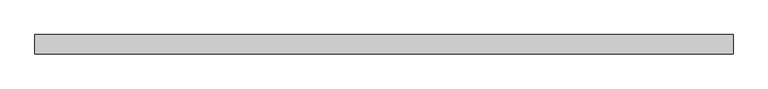
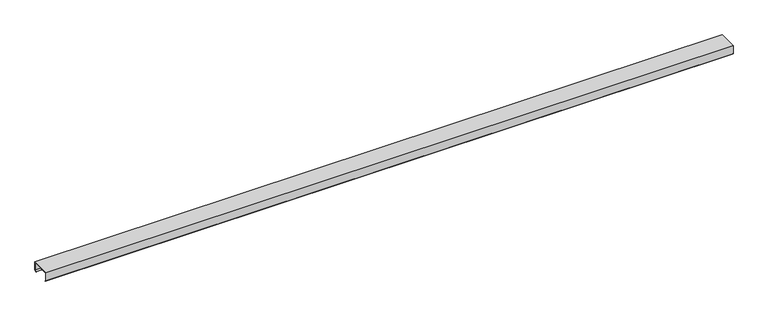
"""IFC4 building model written with IfcOpenShell, lengths in millimetres: proxy geometry, Generic Models 7:Generic Models 1:1:Generic Models 1:1 : Generic Models 7:Generic Models 1:337419:1 : Generic Models 7:Generic Models 1:1:Generic Models 1:1 : Generic Models 7:Generic Models 1:337419:306201."""

from ifc_helpers import new_model, si_unit, frame, origin, place, context, project, spatial, polyline, outline, extrude, source, transform, mapped, element, save


def generic_models_b041f7fe(model_context):
    return source(origin(), model_context, "Body", "SweptSolid", [
        extrude(outline(polyline([(-579000.6913841, 1309.4890625), (-578797.4913841, 1309.4890625), (-578797.4913841, 1220.5890625), (-578812.0845307, 1208.3439586), (-578813.8702751, 1210.4721258), (-578800.2695091, 1221.8845235), (-578800.2695091, 1306.7109375), (-578997.9132591, 1306.7109375), (-578997.9132591, 1221.8845235), (-578984.3124931, 1210.4721258), (-578986.0982375, 1208.3439586), (-579000.6913841, 1220.5890625), (-579000.6913841, 1309.4890625)])), frame((588867.6367239, 0.0, 0.0), z_axis=(1.0, 0.0, 0.0), x_axis=(0.0, 1.0, 0.0)), (0.0, 0.0, 1.0), 7315.2),
    ])


if __name__ == "__main__":
    model = new_model("IFC4")
    model_context = context("Model", 3, world=origin())
    ifc_project = project(units=[si_unit("LENGTHUNIT", "METRE", prefix="MILLI")], contexts=[model_context])
    site = spatial("IfcSite", under=ifc_project)
    building = spatial("IfcBuilding", under=site)
    placement = place(None, origin())
    generic_models_shape = generic_models_b041f7fe(model_context)
    element("IfcBuildingElementProxy", 1, Name="Generic Models 7:Generic Models 1:1:Generic Models 1:1 : Generic Models 7:Generic Models 1:337419:1 : Generic Models 7:Generic Models 1:1:Generic Models 1:1 : Generic Models 7:Generic Models 1:337419:306201", ObjectType="Generic Models 7:Generic Models 1:1:Generic Models 1:1 : Generic Models 7:Generic Models 1:337419:1 : Generic Models 7:Generic Models 1:1:Generic Models 1:1 : Generic Models 7:Generic Models 1:337419:306201", at=placement, inside=building, context=model_context, shape_type="MappedRepresentation", body=[
        mapped(generic_models_shape, transform((0.0, 0.0, 0.0), x_axis=(1.0, 0.0, 0.0), y_axis=(0.0, 1.0, 0.0), z_axis=(0.0, 0.0, 1.0))),
    ])
    save(model, "model.ifc")

# Revit data of these elements
# Type "Generic Models 7:Generic Models 1:1:Generic Models 1:1 : Generic Models 7:Generic Models 1:337419:1 : Generic Models 7:Generic Models 1:1:Generic Models 1:1 : Generic Models 7:Generic Models 1:337419:306201"
#   NameOverride = "Generic Models 7:Generic Models 1:1:Generic Models 1:1 : Generic Models 7:Generic Models 1:337419:306201"
#   ObjectTypeOverride = "Generic Models 1:1 : Generic Models 7:Generic Models 1:337419"
#   Reference = "Generic Models 1"
#   Tag = "306201"
# Element 1 (IfcBuildingElementProxy, "Generic Models 7:Generic Models 1:1:Generic Models 1:1 : Generic Models 7:Generic Models 1:337419:1 : Generic Models 7:Generic Models 1:1:Generic Models 1:1 : Generic Models 7:Generic Models 1:337419:306201")
#   Materials on its faces: "CEE' SECTION (8.0x3.5C - SEE STRUCT. DWGS)"
# Materials
#   "CEE' SECTION (8.0x3.5C - SEE STRUCT. DWGS)": class "Unassigned", colour RGB 210 209 208, transparency 0, Keynote = "M05121300.02", Cost = 0
